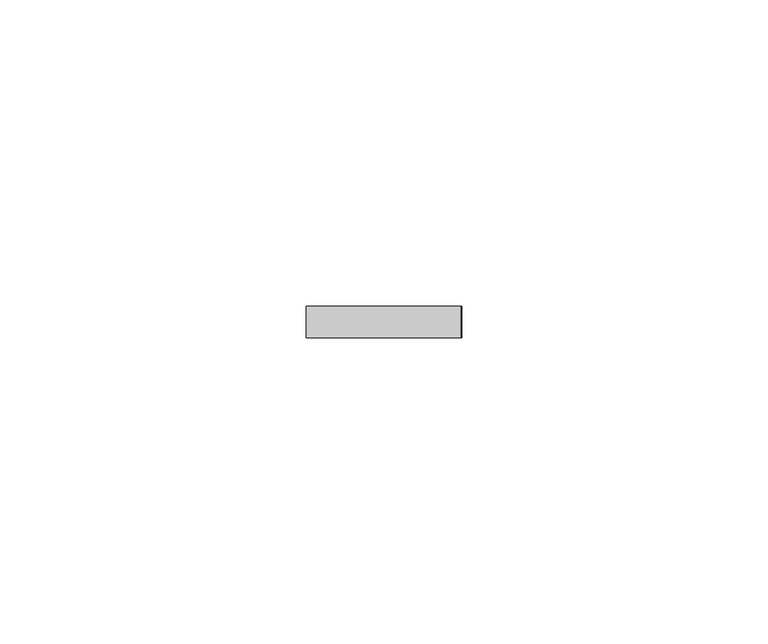
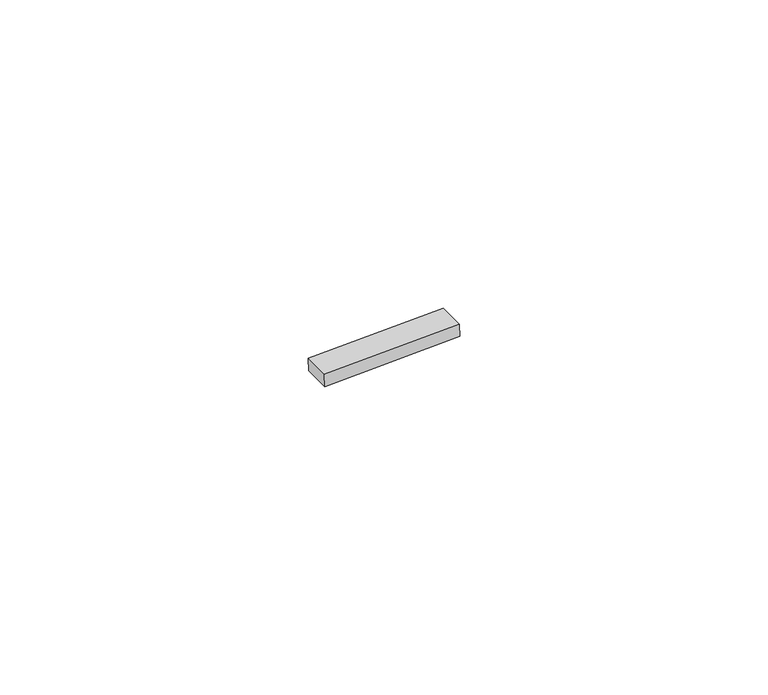
"""IFC4 building model written with IfcOpenShell, lengths in millimetres: proxy geometry, Inner panel:Inner panel:1:Inner panel:1 : Inner panel:Inner panel:300324:2:Inner panel:1:Inner panel:1 : Inner panel:Inner panel:300324:2 : Inner panel:Inner panel:1:Inner panel:1 : Inner panel:Inner panel:300324:300043:170 : Inner panel:Inner panel:1:Inner panel:1 : Inner panel:Inner panel:300324:2:Inner panel:1:Inner panel:1 : Inner panel:Inner panel:300324:2 : Inner panel:Inner panel:1:Inner panel:1 : Inner panel:Inner panel:300324:300043:308120."""

from ifc_helpers import new_model, si_unit, frame, origin, place, context, project, spatial, polyline, outline, extrude, source, transform, mapped, element, save


def generic_models_69b3451e(model_context):
    return source(origin(), model_context, "Body", "SweptSolid", [
        extrude(outline(polyline([(0.0, -25.4), (0.0, 0.0), (5.213809, 0.0), (5.213809, -25.4), (0.0, -25.4)])), frame((560380.9331581, -564587.707991, 3950.5346612), z_axis=(-0.041630544712223896, 0.0, 0.9991330730923502), x_axis=(0.0, -1.0, 0.0)), (0.0, 0.0, 1.0), 2.4763745),
    ])


if __name__ == "__main__":
    model = new_model("IFC4")
    model_context = context("Model", 3, world=origin())
    ifc_project = project(units=[si_unit("LENGTHUNIT", "METRE", prefix="MILLI")], contexts=[model_context])
    site = spatial("IfcSite", under=ifc_project)
    building = spatial("IfcBuilding", under=site)
    placement = place(None, origin())
    generic_models_shape = generic_models_69b3451e(model_context)
    element("IfcBuildingElementProxy", 1, Name="Inner panel:Inner panel:1:Inner panel:1 : Inner panel:Inner panel:300324:2:Inner panel:1:Inner panel:1 : Inner panel:Inner panel:300324:2 : Inner panel:Inner panel:1:Inner panel:1 : Inner panel:Inner panel:300324:300043:170 : Inner panel:Inner panel:1:Inner panel:1 : Inner panel:Inner panel:300324:2:Inner panel:1:Inner panel:1 : Inner panel:Inner panel:300324:2 : Inner panel:Inner panel:1:Inner panel:1 : Inner panel:Inner panel:300324:300043:308120", ObjectType="Inner panel:Inner panel:1:Inner panel:1 : Inner panel:Inner panel:300324:2:Inner panel:1:Inner panel:1 : Inner panel:Inner panel:300324:2 : Inner panel:Inner panel:1:Inner panel:1 : Inner panel:Inner panel:300324:300043:170 : Inner panel:Inner panel:1:Inner panel:1 : Inner panel:Inner panel:300324:2:Inner panel:1:Inner panel:1 : Inner panel:Inner panel:300324:2 : Inner panel:Inner panel:1:Inner panel:1 : Inner panel:Inner panel:300324:300043:308120", at=placement, inside=building, context=model_context, shape_type="MappedRepresentation", body=[
        mapped(generic_models_shape, transform((0.0, 0.0, 0.0), x_axis=(1.0, 0.0, 0.0), y_axis=(0.0, 1.0, 0.0), z_axis=(0.0, 0.0, 1.0))),
    ])
    save(model, "model.ifc")

# Revit data of these elements
# Type "Inner panel:Inner panel:1:Inner panel:1 : Inner panel:Inner panel:300324:2:Inner panel:1:Inner panel:1 : Inner panel:Inner panel:300324:2 : Inner panel:Inner panel:1:Inner panel:1 : Inner panel:Inner panel:300324:300043:170 : Inner panel:Inner panel:1:Inner panel:1 : Inner panel:Inner panel:300324:2:Inner panel:1:Inner panel:1 : Inner panel:Inner panel:300324:2 : Inner panel:Inner panel:1:Inner panel:1 : Inner panel:Inner panel:300324:300043:308120"
#   NameOverride = "Inner panel:Inner panel:1:Inner panel:1 : Inner panel:Inner panel:300324:2:Inner panel:1:Inner panel:1 : Inner panel:Inner panel:300324:2 : Inner panel:Inner panel:1:Inner panel:1 : Inner panel:Inner panel:300324:300043:308120"
#   ObjectTypeOverride = "Inner panel:1:Inner panel:1 : Inner panel:Inner panel:300324:2 : Inner panel:Inner panel:1:Inner panel:1 : Inner panel:Inner panel:300324:300043"
#   Reference = "Inner panel"
#   Tag = "308120"
# Element 1 (IfcBuildingElementProxy, "Inner panel:Inner panel:1:Inner panel:1 : Inner panel:Inner panel:300324:2:Inner panel:1:Inner panel:1 : Inner panel:Inner panel:300324:2 : Inner panel:Inner panel:1:Inner panel:1 : Inner panel:Inner panel:300324:300043:170 : Inner panel:Inner panel:1:Inner panel:1 : Inner panel:Inner panel:300324:2:Inner panel:1:Inner panel:1 : Inner panel:Inner panel:300324:2 : Inner panel:Inner panel:1:Inner panel:1 : Inner panel:Inner panel:300324:300043:308120")
#   Materials on its faces: "AT CLIP - 1\" WIDE NON ABSORBENT, WEATHER-RESISTANT NEOPRENE/EPDM/SBR FOAM"
# Materials
#   "AT CLIP - 1\" WIDE NON ABSORBENT, WEATHER-RESISTANT NEOPRENE/EPDM/SBR FOAM": class "Generic", colour RGB 85 85 85, transparency 0, Cost = 0
